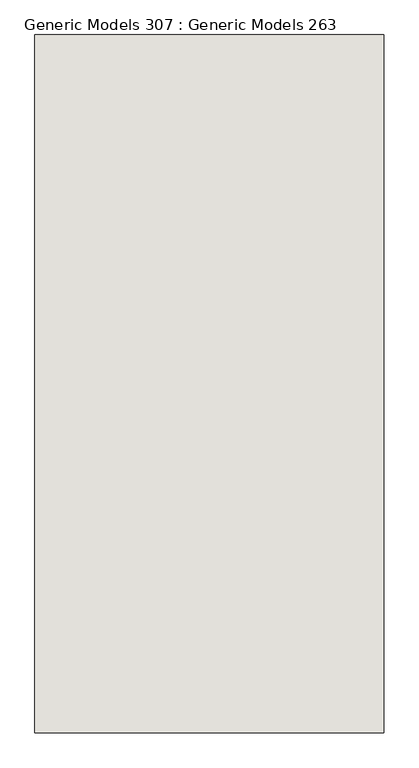
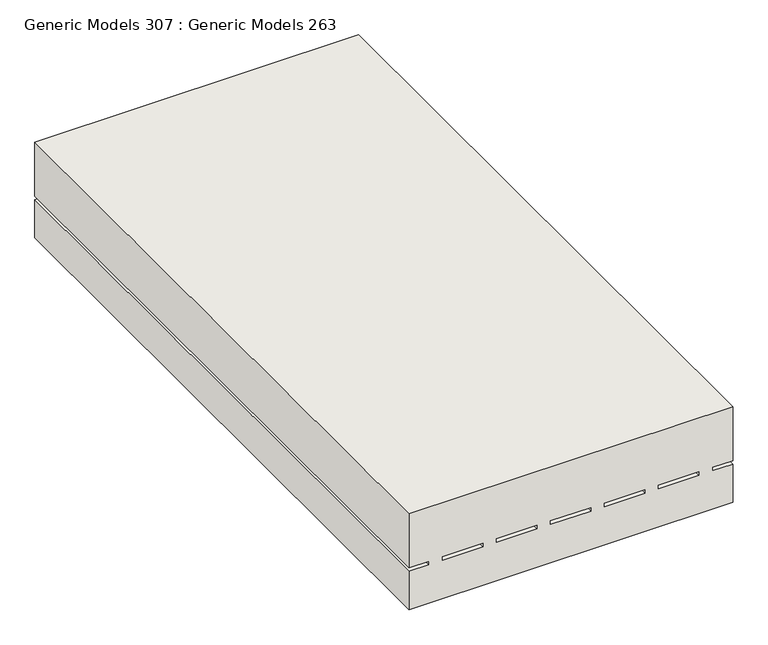
"""IFC4 building model written with IfcOpenShell, lengths in millimetres: wall geometry, Generic Models 307 : Generic Models 263."""

from ifc_helpers import new_model, si_unit, frame, origin, place, context, project, spatial, polyline, outline, extrude, source, transform, mapped, element, save


def generic_models_307_generic_models_263_524330a5(model_context):
    return source(origin(), model_context, "Body", "SweptSolid", [
        extrude(outline(polyline([(0.0, 95516.9797726), (0.0, 94907.3797726), (-107.2982847, 94907.3797726), (-107.2982847, 94945.4797726), (-114.3, 94945.4797726), (-114.3, 94907.3797726), (-190.5, 94907.3797726), (-190.5, 95516.9797726), (-114.3, 95516.9797726), (-114.3, 95478.8797726), (-107.2982847, 95478.8797726), (-107.2982847, 95516.9797726), (0.0, 95516.9797726)]), holes=[polyline([(-107.2982847, 94970.8797726), (-107.2982847, 95047.0797726), (-114.3, 95047.0797726), (-114.3, 94970.8797726), (-107.2982847, 94970.8797726)]), polyline([(-107.2982847, 95072.4797726), (-107.2982847, 95148.6797726), (-114.3, 95148.6797726), (-114.3, 95072.4797726), (-107.2982847, 95072.4797726)]), polyline([(-107.2982847, 95174.0797726), (-107.2982847, 95250.2797726), (-114.3, 95250.2797726), (-114.3, 95174.0797726), (-107.2982847, 95174.0797726)]), polyline([(-107.2982847, 95275.6797726), (-107.2982847, 95351.8797726), (-114.3, 95351.8797726), (-114.3, 95275.6797726), (-107.2982847, 95275.6797726)]), polyline([(-107.2982847, 95377.2797726), (-107.2982847, 95453.4797726), (-114.3, 95453.4797726), (-114.3, 95377.2797726), (-107.2982847, 95377.2797726)])]), frame((0.0, -94.4486541, 0.0), z_axis=(0.0, 1.0, 0.0), x_axis=(0.0, 0.0, 1.0)), (0.0, 0.0, 1.0), 1219.2),
    ])


if __name__ == "__main__":
    model = new_model("IFC4")
    model_context = context("Model", 3, world=origin())
    ifc_project = project(units=[si_unit("LENGTHUNIT", "METRE", prefix="MILLI")], contexts=[model_context])
    site = spatial("IfcSite", under=ifc_project)
    building = spatial("IfcBuilding", under=site)
    placement = place(None, origin())
    generic_models_307_generic_models_263_shape = generic_models_307_generic_models_263_524330a5(model_context)
    element("IfcWall", 1, ObjectType="Generic Models 307 : Generic Models 263", at=placement, inside=building, context=model_context, shape_type="MappedRepresentation", body=[
        mapped(generic_models_307_generic_models_263_shape, transform((0.0, 0.0, 0.0), x_axis=(1.0, 0.0, 0.0), y_axis=(0.0, 1.0, 0.0), z_axis=(0.0, 0.0, 1.0))),
    ])
    save(model, "model.ifc")

# Revit data of these elements
# Element 1 (IfcWall, "Generic Models 307 : Generic Models 263")
#   Materials on its faces: "CONCRETE PAVEMENT HEAVY DUTY"
# Materials
#   "CONCRETE PAVEMENT HEAVY DUTY": class "Concrete", colour RGB 191 191 191, transparency 0, Description = "Cast-in-place concrete", Cost = 0
